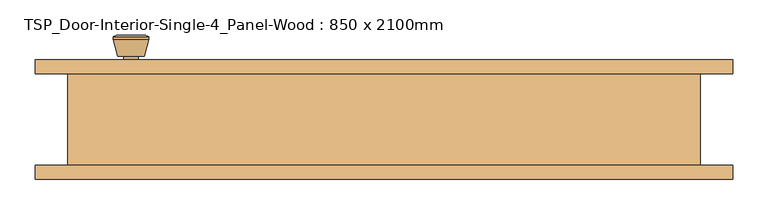
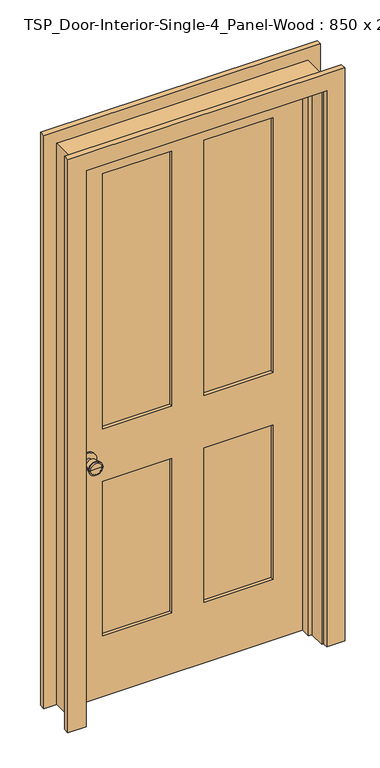
"""IFC4 building model written with IfcOpenShell, lengths in millimetres: door geometry, TSP_Door-Interior-Single-4_Panel-Wood : 850 x 2100mm."""

import ifcopenshell
import ifcopenshell.guid

model = None  # the IFC model being written
_history = None  # IfcOwnerHistory: only IFC2X3 demands one
_inside = {}  # id of a spatial element -> (the spatial element, [elements in it])
_under = {}  # id of a project, library or spatial element -> (it, [spatial elements below it])
_declared = {}  # id of a project -> (the project, [libraries it declares])
_typed = {}  # id of a type object -> (the type object, [elements of that type])
_made_of = {}  # id of a material, layer set ... -> (it, [elements and type objects made of it])


def new_model(schema):
    """Start an empty IFC model of exactly this schema.

    Asked for "IFC4X3", IfcOpenShell would pick the latest addendum, in which some entities
    have other attributes; the version numbers below select the first issue.
    IFC2X3 requires an IfcOwnerHistory on every rooted entity: one is made here for all.
    """
    global model, _history
    if schema == "IFC4X3":
        model = ifcopenshell.file(schema_version=(4, 3, 0, 0))
    else:
        model = ifcopenshell.file(schema=schema)
    _inside.clear()
    _under.clear()
    _declared.clear()
    _typed.clear()
    _made_of.clear()
    _history = None
    if model.schema == "IFC2X3":
        org = make("IfcOrganization", Name="unknown")
        user = make(
            "IfcPersonAndOrganization",
            ThePerson=make("IfcPerson", FamilyName="unknown"),
            TheOrganization=org,
        )
        app = make(
            "IfcApplication",
            ApplicationDeveloper=org,
            Version="unknown",
            ApplicationFullName="unknown",
            ApplicationIdentifier="unknown",
        )
        _history = make(
            "IfcOwnerHistory",
            OwningUser=user,
            OwningApplication=app,
            ChangeAction="ADDED",
            CreationDate=0,
        )
    return model


def make(cls, **values):
    """One entity of the class cls with the attributes given. An attribute that is None is left unset."""
    return model.create_entity(
        cls, **{name: value for name, value in values.items() if value is not None}
    )


def rooted(cls, **values):
    """An entity with a GlobalId (a new one), such as an element, a storey or a relation."""
    return make(cls, GlobalId=ifcopenshell.guid.new(), OwnerHistory=_history, **values)


def si_unit(unit_type, name, prefix=None):
    """IfcSIUnit, for example si_unit("LENGTHUNIT", "METRE", prefix="MILLI")."""
    return make("IfcSIUnit", UnitType=unit_type, Prefix=prefix, Name=name)


def assignment(units):
    """IfcUnitAssignment: the units of a project."""
    return None if units is None else make("IfcUnitAssignment", Units=units)


def point(xyz):
    """IfcCartesianPoint."""
    return None if xyz is None else make("IfcCartesianPoint", Coordinates=xyz)


def direction(xyz):
    """IfcDirection."""
    return None if xyz is None else make("IfcDirection", DirectionRatios=xyz)


def frame(location, z_axis=None, x_axis=None):
    """IfcAxis2Placement3D, a coordinate frame: its origin and axes. An axis left out is left unset."""
    return make(
        "IfcAxis2Placement3D",
        Location=point(location),
        Axis=direction(z_axis),
        RefDirection=direction(x_axis),
    )


def frame_2d(location, x_axis=None):
    """IfcAxis2Placement2D, a coordinate frame in the plane: its origin and x axis."""
    return make(
        "IfcAxis2Placement2D", Location=point(location), RefDirection=direction(x_axis)
    )


def origin():
    """The frame at (0, 0, 0) with its axes left unset."""
    return frame((0.0, 0.0, 0.0))


def place(relative_to, where):
    """IfcLocalPlacement: puts the frame where relative to a parent placement (None: the world)."""
    return make(
        "IfcLocalPlacement", PlacementRelTo=relative_to, RelativePlacement=where
    )


def context(
    kind, dimensions, precision=None, world=None, true_north=None, identifier=None
):
    """IfcGeometricRepresentationContext, for example the 3D "Model" context."""
    return make(
        "IfcGeometricRepresentationContext",
        ContextIdentifier=identifier,
        ContextType=kind,
        CoordinateSpaceDimension=dimensions,
        Precision=precision,
        WorldCoordinateSystem=world,
        TrueNorth=true_north,
    )


def project(units=None, contexts=None):
    """IfcProject with its units and contexts."""
    return rooted(
        "IfcProject",
        Name="project",
        RepresentationContexts=contexts,
        UnitsInContext=assignment(units),
    )


def spatial(cls, under=None, at=None, **own):
    """A site, building, storey or space (cls), placed at a placement, below another one or the project."""
    s = rooted(cls, ObjectPlacement=at, **own)
    if under is not None:
        _under.setdefault(under.id(), (under, []))[1].append(s)
    return s


def polyline(points):
    """IfcPolyline through the points."""
    return make("IfcPolyline", Points=[point(p) for p in points])


def circle_curve(where, radius):
    """IfcCircle in the frame where."""
    return make("IfcCircle", Position=where, Radius=radius)


def trimmed(basis, trim1, trim2, sense, master):
    """IfcTrimmedCurve: the piece of a basis curve between two trims."""
    return make(
        "IfcTrimmedCurve",
        BasisCurve=basis,
        Trim1=trim1,
        Trim2=trim2,
        SenseAgreement=sense,
        MasterRepresentation=master,
    )


def segment(curve, same_sense, transition):
    """IfcCompositeCurveSegment."""
    return make(
        "IfcCompositeCurveSegment",
        Transition=transition,
        SameSense=same_sense,
        ParentCurve=curve,
    )


def composite_curve(segments, self_intersect=None):
    """IfcCompositeCurve: segments joined end to end."""
    return make("IfcCompositeCurve", Segments=segments, SelfIntersect=self_intersect)


def outline(outer, holes=None, kind="AREA"):
    """IfcArbitraryClosedProfileDef: a profile drawn as a closed curve; with holes, ...WithVoids."""
    if holes is None:
        return make("IfcArbitraryClosedProfileDef", ProfileType=kind, OuterCurve=outer)
    return make(
        "IfcArbitraryProfileDefWithVoids",
        ProfileType=kind,
        OuterCurve=outer,
        InnerCurves=holes,
    )


def extrude(swept, where, along, depth):
    """IfcExtrudedAreaSolid: the profile swept, set in the frame where, extruded along a direction by depth."""
    return make(
        "IfcExtrudedAreaSolid",
        SweptArea=swept,
        Position=where,
        ExtrudedDirection=direction(along),
        Depth=depth,
    )


def faces_of(points, faces, orient=None, outer=None):
    """IfcFace entities. A face is a list of loops; a loop is a list of indices into points, from 0.

    orient and outer hold one flag for each loop. By default every Orientation is true, the
    first loop of a face is its IfcFaceOuterBound and the others are IfcFaceBound.
    """
    made = []
    for i, loops in enumerate(faces):
        bounds = []
        for j, loop in enumerate(loops):
            is_outer = j == 0 if outer is None else outer[i][j]
            bounds.append(
                make(
                    "IfcFaceOuterBound" if is_outer else "IfcFaceBound",
                    Bound=make("IfcPolyLoop", Polygon=[points[k] for k in loop]),
                    Orientation=True if orient is None else orient[i][j],
                )
            )
        made.append(make("IfcFace", Bounds=bounds))
    return made


def faceted_brep(points, faces, orient=None, outer=None, voids=None):
    """IfcFacetedBrep: a solid bounded by flat faces; with voids (closed shells), ...WithVoids."""
    shared = [point(p) for p in points]
    hull = make("IfcClosedShell", CfsFaces=faces_of(shared, faces, orient, outer))
    if voids is None:
        return make("IfcFacetedBrep", Outer=hull)
    return make(
        "IfcFacetedBrepWithVoids",
        Outer=hull,
        Voids=[
            make(cls, CfsFaces=faces_of(shared, fs, o, b)) for cls, fs, o, b in voids
        ],
    )


def shape(context_of_items, identifier, shape_type, items):
    """IfcShapeRepresentation: the items that make up one representation, for example the "Body"."""
    return make(
        "IfcShapeRepresentation",
        ContextOfItems=context_of_items,
        RepresentationIdentifier=identifier,
        RepresentationType=shape_type,
        Items=items,
    )


def source(mapping_origin, context_of_items, identifier, shape_type, items):
    """IfcRepresentationMap: a shape defined once, which mapped items show again and again."""
    return make(
        "IfcRepresentationMap",
        MappingOrigin=mapping_origin,
        MappedRepresentation=shape(context_of_items, identifier, shape_type, items),
    )


def transform(
    local_origin,
    x_axis=None,
    y_axis=None,
    z_axis=None,
    scale=None,
    scale2=None,
    scale3=None,
    uniform=True,
):
    """IfcCartesianTransformationOperator3D, or its non-uniform kind. x_axis, y_axis, z_axis: its Axis1, 2, 3."""
    if uniform:
        return make(
            "IfcCartesianTransformationOperator3D",
            Axis1=direction(x_axis),
            Axis2=direction(y_axis),
            LocalOrigin=point(local_origin),
            Scale=scale,
            Axis3=direction(z_axis),
        )
    return make(
        "IfcCartesianTransformationOperator3DnonUniform",
        Axis1=direction(x_axis),
        Axis2=direction(y_axis),
        LocalOrigin=point(local_origin),
        Scale=scale,
        Axis3=direction(z_axis),
        Scale2=scale2,
        Scale3=scale3,
    )


def mapped(mapping_source, mapping_target):
    """IfcMappedItem: shows the shape of a source again, moved by a transform."""
    return make(
        "IfcMappedItem", MappingSource=mapping_source, MappingTarget=mapping_target
    )


def made_of(thing, what):
    """Note that an element or type object is made of a material, layer set ...; save() writes the relation."""
    if what is not None:
        _made_of.setdefault(what.id(), (what, []))[1].append(thing)
    return thing


def element(
    cls,
    number,
    at=None,
    inside=None,
    cuts=None,
    type_object=None,
    material=None,
    context=None,
    identifier="Body",
    shape_type=None,
    held_by="IfcProductDefinitionShape",
    body=None,
    shapes=None,
    **own,
):
    """One element of the class cls, such as IfcWall. Its Tag is "e" and its number.

    at: its placement. inside: the storey or other place that contains it. cuts: it is an
    opening in that element (IfcRelVoidsElement). A single representation is given by context,
    identifier, shape_type and body (its items); several are given by shapes. held_by: the class
    of the entity that holds the representations. save() writes the other relations.
    """
    e = rooted(cls, Tag="e%d" % number, ObjectPlacement=at, **own)
    if body is not None:
        shapes = [shape(context, identifier, shape_type, body)]
    if shapes is not None:
        e.Representation = make(held_by, Representations=shapes)
    if inside is not None:
        _inside.setdefault(inside.id(), (inside, []))[1].append(e)
    if cuts is not None:
        rooted(
            "IfcRelVoidsElement", RelatingBuildingElement=cuts, RelatedOpeningElement=e
        )
    if type_object is not None:
        _typed.setdefault(type_object.id(), (type_object, []))[1].append(e)
    return made_of(e, material)


def aggregate(whole, parts):
    """IfcRelAggregates: a whole, such as a stair, and the parts it consists of."""
    return rooted("IfcRelAggregates", RelatingObject=whole, RelatedObjects=parts)


def save(model, path):
    """Write the relations noted so far, then the file.

    IfcRelAggregates (storeys below a building ...), IfcRelContainedInSpatialStructure (elements
    in a storey), IfcRelDefinesByType, IfcRelAssociatesMaterial and IfcRelDeclares: one each for
    every whole, place, type object, material and project.
    """
    for whole, parts in _under.values():
        aggregate(whole, parts)
    for where, things in _inside.values():
        rooted(
            "IfcRelContainedInSpatialStructure",
            RelatedElements=things,
            RelatingStructure=where,
        )
    for kind, things in _typed.values():
        rooted("IfcRelDefinesByType", RelatedObjects=things, RelatingType=kind)
    for what, things in _made_of.values():
        rooted("IfcRelAssociatesMaterial", RelatedObjects=things, RelatingMaterial=what)
    for by, libraries in _declared.values():
        rooted("IfcRelDeclares", RelatingContext=by, RelatedDefinitions=libraries)
    model.write(path)


def plane_surface(at):
    """IfcPlane: the flat surface through the origin of the frame at, square to its z axis."""
    return make("IfcPlane", Position=at)


def cylinder_surface(at, radius):
    """IfcCylindricalSurface: all points at the distance radius from the z axis of the frame at."""
    return make("IfcCylindricalSurface", Position=at, Radius=radius)


def revolved_surface(curve, axis_point, axis_direction):
    """IfcSurfaceOfRevolution: the curve turned about the line through axis_point along axis_direction."""
    return make(
        "IfcSurfaceOfRevolution",
        SweptCurve=make("IfcArbitraryOpenProfileDef", ProfileType="CURVE", Curve=curve),
        AxisPosition=make("IfcAxis1Placement", Location=point(axis_point), Axis=direction(axis_direction)),
    )


def advanced_brep(points, edges, surfaces, faces):
    """IfcAdvancedBrep: a solid bounded by faces that lie on surfaces and meet in shared edges.

    An edge is (start, end): straight between two places in points (the first is 0);
    or (start, end, curve); or (start, end, curve, False) where it runs against its curve.
    A face is (place in surfaces, loops), or (place, loops, False) where it looks against
    its surface's normal. A loop lists edges by number (the first is 1), with a minus sign
    where the edge is run from its end to its start. The first loop is the outer one.
    """
    corners = [point(p) for p in points]
    vertices = [make("IfcVertexPoint", VertexGeometry=c) for c in corners]
    made = []
    for start, end, *more in edges:
        made.append(
            make(
                "IfcEdgeCurve",
                EdgeStart=vertices[start],
                EdgeEnd=vertices[end],
                EdgeGeometry=more[0] if more else make("IfcPolyline", Points=[corners[start], corners[end]]),
                SameSense=more[1] if len(more) > 1 else True,
            )
        )
    hull = []
    for where, loops, *sense in faces:
        bounds = []
        for j, loop in enumerate(loops):
            ring = [make("IfcOrientedEdge", EdgeElement=made[abs(k) - 1], Orientation=k > 0) for k in loop]
            bounds.append(
                make(
                    "IfcFaceOuterBound" if j == 0 else "IfcFaceBound",
                    Bound=make("IfcEdgeLoop", EdgeList=ring),
                    Orientation=True,
                )
            )
        hull.append(make("IfcAdvancedFace", Bounds=bounds, FaceSurface=surfaces[where], SameSense=sense[0] if sense else True))
    return make("IfcAdvancedBrep", Outer=make("IfcClosedShell", CfsFaces=hull))


def tsp_door_interior_single_4_panel_wood_850_x_2100mm_ed8611a6(model_context):
    return source(origin(), model_context, "Body", "SolidModel", [
        advanced_brep(
        [(-360.0, 20.825, 914.4), (-350.0, 20.825, 914.4), (-370.0, 20.825, 914.4), (-339.5241324, -28.175, 914.4), (-360.0, -28.175, 914.4), (-380.4758676, -28.175, 914.4), (-335.0, -26.3471319, 914.4), (-385.0, -26.3471319, 914.4), (-335.0, -22.8834537, 914.4), (-385.0, -22.8834537, 914.4), (-341.363764, 1.825, 914.4), (-378.636236, 1.825, 914.4), (-350.0, 1.825, 914.4), (-370.0, 1.825, 914.4)],
        [
            (0, 1),
            (1, 2, circle_curve(frame((-360.0, 20.825, 914.4), z_axis=(0.0, 1.0, 0.0), x_axis=(-1.0, 0.0, 0.0)), 10.0)),
            (2, 0),
            (2, 1, circle_curve(frame((-360.0, 20.825, 914.4), z_axis=(0.0, 1.0, 0.0), x_axis=(-1.0, 0.0, 0.0)), 10.0)),
            (3, 4),
            (4, 5),
            (5, 3, circle_curve(frame((-360.0, -28.175, 914.4), z_axis=(0.0, -1.0, 0.0), x_axis=(-1.0, 0.0, 0.0)), 20.4758676)),
            (3, 5, circle_curve(frame((-360.0, -28.175, 914.4), z_axis=(0.0, -1.0, 0.0), x_axis=(-1.0, 0.0, 0.0)), 20.4758676)),
            (6, 3),
            (5, 7),
            (7, 6, circle_curve(frame((-360.0, -26.3471319, 914.4), z_axis=(0.0, -1.0, 0.0), x_axis=(-1.0, 0.0, 0.0)), 25.0)),
            (6, 7, circle_curve(frame((-360.0, -26.3471319, 914.4), z_axis=(0.0, -1.0, 0.0), x_axis=(-1.0, 0.0, 0.0)), 25.0)),
            (8, 6),
            (7, 9),
            (9, 8, circle_curve(frame((-360.0, -22.8834537, 914.4), z_axis=(0.0, -1.0, 0.0), x_axis=(-1.0, 0.0, 0.0)), 25.0)),
            (8, 9, circle_curve(frame((-360.0, -22.8834537, 914.4), z_axis=(0.0, -1.0, 0.0), x_axis=(-1.0, 0.0, 0.0)), 25.0)),
            (10, 8),
            (9, 11),
            (11, 10, circle_curve(frame((-360.0, 1.825, 914.4), z_axis=(0.0, -1.0, 0.0), x_axis=(-1.0, 0.0, 0.0)), 18.636236)),
            (10, 11, circle_curve(frame((-360.0, 1.825, 914.4), z_axis=(0.0, -1.0, 0.0), x_axis=(-1.0, 0.0, 0.0)), 18.636236)),
            (12, 10),
            (11, 13),
            (13, 12, circle_curve(frame((-360.0, 1.825, 914.4), z_axis=(0.0, -1.0, 0.0), x_axis=(-1.0, 0.0, 0.0)), 10.0)),
            (12, 13, circle_curve(frame((-360.0, 1.825, 914.4), z_axis=(0.0, -1.0, 0.0), x_axis=(-1.0, 0.0, 0.0)), 10.0)),
            (1, 12),
            (13, 2),
        ],
        [
            plane_surface(frame((-360.0, 20.825, 914.4), z_axis=(0.0, 1.0, 0.0), x_axis=(-1.0, 0.0, 0.0))),
            plane_surface(frame((-360.0, -28.175, 914.4), z_axis=(0.0, -1.0, 0.0), x_axis=(-1.0, 0.0, 0.0))),
            revolved_surface(polyline([(-380.4758676, -28.175, 914.4), (-385.0, -26.3471319, 914.4)]), (-360.0, 20.825, 914.4), (0.0, 1.0, 0.0)),
            cylinder_surface(frame((-360.0, 20.825, 914.4), z_axis=(0.0, 1.0, 0.0), x_axis=(-1.0, 0.0, 0.0)), 25.0),
            revolved_surface(polyline([(-385.0, -22.8834537, 914.4), (-378.636236, 1.825, 914.4)]), (-360.0, 20.825, 914.4), (0.0, 1.0, 0.0)),
            plane_surface(frame((-360.0, 1.825, 914.4), z_axis=(0.0, 1.0, 0.0), x_axis=(-1.0, 0.0, 0.0))),
            cylinder_surface(frame((-360.0, 20.825, 914.4), z_axis=(0.0, 1.0, 0.0), x_axis=(-1.0, 0.0, 0.0)), 10.0),
        ],
        [
            (0, [[1, 2, 3]]),
            (0, [[-3, 4, -1]]),
            (1, [[5, 6, 7]]),
            (1, [[-6, -5, 8]]),
            (2, [[9, -7, 10, 11]]),
            (2, [[-10, -8, -9, 12]]),
            (3, [[13, -11, 14, 15]]),
            (3, [[-14, -12, -13, 16]]),
            (4, [[17, -15, 18, 19]]),
            (4, [[-18, -16, -17, 20]]),
            (5, [[21, -19, 22, 23]]),
            (5, [[-22, -20, -21, 24]]),
            (6, [[25, -23, 26, -2]]),
            (6, [[-26, -24, -25, -4]]),
        ],
    ),
        extrude(outline(composite_curve([segment(trimmed(circle_curve(frame_2d((914.4, -360.0)), 30.0), [point((914.4, -390.0))], [point((914.4, -330.0))], False, "CARTESIAN"), True, "CONTINUOUS"), segment(trimmed(circle_curve(frame_2d((914.4, -360.0)), 30.0), [point((914.4, -330.0))], [point((914.4, -390.0))], False, "CARTESIAN"), True, "CONTINUOUS")], self_intersect=False)), frame((0.0, 20.825, 0.0), z_axis=(0.0, 1.0, 0.0), x_axis=(0.0, 0.0, 1.0)), (0.0, 0.0, 1.0), 6.0),
        advanced_brep(
        [(-360.0, 67.825, 914.4), (-370.0, 67.825, 914.4), (-350.0, 67.825, 914.4), (-339.5241324, 116.825, 914.4), (-380.4758676, 116.825, 914.4), (-360.0, 116.825, 914.4), (-335.0, 114.9971319, 914.4), (-385.0, 114.9971319, 914.4), (-335.0, 111.5334537, 914.4), (-385.0, 111.5334537, 914.4), (-341.363764, 86.825, 914.4), (-378.636236, 86.825, 914.4), (-350.0, 86.825, 914.4), (-370.0, 86.825, 914.4)],
        [
            (0, 1),
            (1, 2, circle_curve(frame((-360.0, 67.825, 914.4), z_axis=(0.0, -1.0, 0.0), x_axis=(-1.0, 0.0, 0.0)), 10.0)),
            (2, 0),
            (2, 1, circle_curve(frame((-360.0, 67.825, 914.4), z_axis=(0.0, -1.0, 0.0), x_axis=(-1.0, 0.0, 0.0)), 10.0)),
            (3, 4, circle_curve(frame((-360.0, 116.825, 914.4), z_axis=(0.0, 1.0, 0.0), x_axis=(-1.0, 0.0, 0.0)), 20.4758676)),
            (4, 5),
            (5, 3),
            (4, 3, circle_curve(frame((-360.0, 116.825, 914.4), z_axis=(0.0, 1.0, 0.0), x_axis=(-1.0, 0.0, 0.0)), 20.4758676)),
            (6, 7, circle_curve(frame((-360.0, 114.9971319, 914.4), z_axis=(0.0, 1.0, 0.0), x_axis=(-1.0, 0.0, 0.0)), 25.0)),
            (7, 4),
            (3, 6),
            (7, 6, circle_curve(frame((-360.0, 114.9971319, 914.4), z_axis=(0.0, 1.0, 0.0), x_axis=(-1.0, 0.0, 0.0)), 25.0)),
            (8, 9, circle_curve(frame((-360.0, 111.5334537, 914.4), z_axis=(0.0, 1.0, 0.0), x_axis=(-1.0, 0.0, 0.0)), 25.0)),
            (9, 7),
            (6, 8),
            (9, 8, circle_curve(frame((-360.0, 111.5334537, 914.4), z_axis=(0.0, 1.0, 0.0), x_axis=(-1.0, 0.0, 0.0)), 25.0)),
            (10, 11, circle_curve(frame((-360.0, 86.825, 914.4), z_axis=(0.0, 1.0, 0.0), x_axis=(-1.0, 0.0, 0.0)), 18.636236)),
            (11, 9),
            (8, 10),
            (11, 10, circle_curve(frame((-360.0, 86.825, 914.4), z_axis=(0.0, 1.0, 0.0), x_axis=(-1.0, 0.0, 0.0)), 18.636236)),
            (12, 13, circle_curve(frame((-360.0, 86.825, 914.4), z_axis=(0.0, 1.0, 0.0), x_axis=(-1.0, 0.0, 0.0)), 10.0)),
            (13, 11),
            (10, 12),
            (13, 12, circle_curve(frame((-360.0, 86.825, 914.4), z_axis=(0.0, 1.0, 0.0), x_axis=(-1.0, 0.0, 0.0)), 10.0)),
            (1, 13),
            (12, 2),
        ],
        [
            plane_surface(frame((-360.0, 67.825, 914.4), z_axis=(0.0, -1.0, 0.0), x_axis=(-1.0, 0.0, 0.0))),
            plane_surface(frame((-360.0, 116.825, 914.4), z_axis=(0.0, 1.0, 0.0), x_axis=(-1.0, 0.0, 0.0))),
            revolved_surface(polyline([(-380.4758676, 116.825, 914.4), (-385.0, 114.9971319, 914.4)]), (-360.0, 67.825, 914.4), (0.0, -1.0, 0.0)),
            cylinder_surface(frame((-360.0, 67.825, 914.4), z_axis=(0.0, -1.0, 0.0), x_axis=(-1.0, 0.0, 0.0)), 25.0),
            revolved_surface(polyline([(-385.0, 111.5334537, 914.4), (-378.636236, 86.825, 914.4)]), (-360.0, 67.825, 914.4), (0.0, -1.0, 0.0)),
            plane_surface(frame((-360.0, 86.825, 914.4), z_axis=(0.0, -1.0, 0.0), x_axis=(-1.0, 0.0, 0.0))),
            cylinder_surface(frame((-360.0, 67.825, 914.4), z_axis=(0.0, -1.0, 0.0), x_axis=(-1.0, 0.0, 0.0)), 10.0),
        ],
        [
            (0, [[1, 2, 3]]),
            (0, [[-3, 4, -1]]),
            (1, [[5, 6, 7]]),
            (1, [[8, -7, -6]]),
            (2, [[9, 10, -5, 11]]),
            (2, [[12, -11, -8, -10]]),
            (3, [[13, 14, -9, 15]]),
            (3, [[16, -15, -12, -14]]),
            (4, [[17, 18, -13, 19]]),
            (4, [[20, -19, -16, -18]]),
            (5, [[21, 22, -17, 23]]),
            (5, [[24, -23, -20, -22]]),
            (6, [[-2, 25, -21, 26]]),
            (6, [[-4, -26, -24, -25]]),
        ],
    ),
        extrude(outline(composite_curve([segment(trimmed(circle_curve(frame_2d((914.4, -360.0)), 30.0), [point((914.4, -390.0))], [point((914.4, -330.0))], False, "CARTESIAN"), True, "CONTINUOUS"), segment(trimmed(circle_curve(frame_2d((914.4, -360.0)), 30.0), [point((914.4, -330.0))], [point((914.4, -390.0))], False, "CARTESIAN"), True, "CONTINUOUS")], self_intersect=False)), frame((0.0, 61.825, 0.0), z_axis=(0.0, 1.0, 0.0), x_axis=(0.0, 0.0, 1.0)), (0.0, 0.0, 1.0), 6.0),
        faceted_brep([(450.0, 61.825, 0.0), (450.0, -68.175, 0.0), (425.0, -68.175, 0.0), (425.0, -8.1, 0.0), (412.3, -8.1, 0.0), (412.3, 26.825, 0.0), (425.0, 26.825, 0.0), (425.0, 61.825, 0.0), (450.0, 61.825, 2125.0), (450.0, -68.175, 2125.0), (-450.0, -68.175, 2125.0), (-450.0, -68.175, 0.0), (-425.0, -68.175, 0.0), (-425.0, -68.175, 2100.0), (425.0, -68.175, 2100.0), (425.0, -8.1, 2100.0), (-425.0, -8.1, 2100.0), (-425.0, -8.1, 0.0), (-412.3, -8.1, 0.0), (-412.3, -8.1, 2087.3), (412.3, -8.1, 2087.3), (412.3, 26.825, 2087.3), (-412.3, 26.825, 2087.3), (-412.3, 26.825, 0.0), (-425.0, 26.825, 0.0), (-425.0, 26.825, 2100.0), (425.0, 26.825, 2100.0), (425.0, 61.825, 2100.0), (-425.0, 61.825, 2100.0), (-425.0, 61.825, 0.0), (-450.0, 61.825, 0.0), (-450.0, 61.825, 2125.0)], [[[0, 1, 2, 3, 4, 5, 6, 7]], [[1, 0, 8, 9]], [[2, 1, 9, 10, 11, 12, 13, 14]], [[3, 2, 14, 15]], [[4, 3, 15, 16, 17, 18, 19, 20]], [[5, 4, 20, 21]], [[6, 5, 21, 22, 23, 24, 25, 26]], [[7, 6, 26, 27]], [[0, 7, 27, 28, 29, 30, 31, 8]], [[9, 8, 31, 10]], [[15, 14, 13, 16]], [[21, 20, 19, 22]], [[27, 26, 25, 28]], [[30, 29, 24, 23, 18, 17, 12, 11]], [[10, 31, 30, 11]], [[16, 13, 12, 17]], [[22, 19, 18, 23]], [[28, 25, 24, 29]]]),
        extrude(outline(polyline([(2100.0, -425.0), (0.0, -425.0), (0.0, 425.0), (2100.0, 425.0), (2100.0, -425.0)]), holes=[polyline([(1980.0, 57.5), (1980.0, 305.0), (1014.4, 305.0), (1014.4, 57.5), (1980.0, 57.5)]), polyline([(1014.4, -57.5), (1014.4, -305.0), (1980.0, -305.0), (1980.0, -57.5), (1014.4, -57.5)]), polyline([(814.4, 57.5), (814.4, 305.0), (230.0, 305.0), (230.0, 57.5), (814.4, 57.5)]), polyline([(230.0, -57.5), (230.0, -305.0), (814.4, -305.0), (814.4, -57.5), (230.0, -57.5)])]), frame((0.0, 26.825, 0.0), z_axis=(0.0, 1.0, 0.0), x_axis=(0.0, 0.0, 1.0)), (0.0, 0.0, 1.0), 35.0),
        extrude(outline(polyline([(305.0, 38.4916667), (57.5, 38.4916667), (57.5, 50.1583333), (305.0, 50.1583333), (305.0, 38.4916667)])), frame((0.0, 0.0, 1014.4), z_axis=(0.0, 0.0, 1.0), x_axis=(1.0, 0.0, 0.0)), (0.0, 0.0, 1.0), 965.6),
        extrude(outline(polyline([(-57.5, 38.4916667), (-305.0, 38.4916667), (-305.0, 50.1583333), (-57.5, 50.1583333), (-57.5, 38.4916667)])), frame((0.0, 0.0, 1014.4), z_axis=(0.0, 0.0, 1.0), x_axis=(1.0, 0.0, 0.0)), (0.0, 0.0, 1.0), 965.6),
        extrude(outline(polyline([(305.0, 38.4916667), (57.5, 38.4916667), (57.5, 50.1583333), (305.0, 50.1583333), (305.0, 38.4916667)])), frame((0.0, 0.0, 230.0), z_axis=(0.0, 0.0, 1.0), x_axis=(1.0, 0.0, 0.0)), (0.0, 0.0, 1.0), 584.4),
        extrude(outline(polyline([(-57.5, 38.4916667), (-305.0, 38.4916667), (-305.0, 50.1583333), (-57.5, 50.1583333), (-57.5, 38.4916667)])), frame((0.0, 0.0, 230.0), z_axis=(0.0, 0.0, 1.0), x_axis=(1.0, 0.0, 0.0)), (0.0, 0.0, 1.0), 584.4),
        extrude(outline(polyline([(0.0, 431.35), (0.0, 496.35), (2171.35, 496.35), (2171.35, -496.35), (0.0, -496.35), (0.0, -431.35), (2106.35, -431.35), (2106.35, 431.35), (0.0, 431.35)])), frame((0.0, 61.825, 0.0), z_axis=(0.0, 1.0, 0.0), x_axis=(0.0, 0.0, 1.0)), (0.0, 0.0, 1.0), 20.0),
        extrude(outline(polyline([(0.0, 431.35), (0.0, 496.35), (2171.35, 496.35), (2171.35, -496.35), (0.0, -496.35), (0.0, -431.35), (2106.35, -431.35), (2106.35, 431.35), (0.0, 431.35)])), frame((0.0, -88.175, 0.0), z_axis=(0.0, 1.0, 0.0), x_axis=(0.0, 0.0, 1.0)), (0.0, 0.0, 1.0), 20.0),
    ])


if __name__ == "__main__":
    model = new_model("IFC4")
    model_context = context("Model", 3, world=origin())
    ifc_project = project(units=[si_unit("LENGTHUNIT", "METRE", prefix="MILLI")], contexts=[model_context])
    site = spatial("IfcSite", under=ifc_project)
    building = spatial("IfcBuilding", under=site)
    placement = place(None, origin())
    tsp_door_interior_single_4_panel_wood_850_x_2100mm_shape = tsp_door_interior_single_4_panel_wood_850_x_2100mm_ed8611a6(model_context)
    element("IfcDoor", 1, ObjectType="TSP_Door-Interior-Single-4_Panel-Wood : 850 x 2100mm", at=placement, inside=building, context=model_context, shape_type="MappedRepresentation", body=[
        mapped(tsp_door_interior_single_4_panel_wood_850_x_2100mm_shape, transform((0.0, 0.0, 0.0), x_axis=(1.0, 0.0, 0.0), y_axis=(0.0, 1.0, 0.0), z_axis=(0.0, 0.0, 1.0))),
    ])
    save(model, "model.ifc")

# Revit data of these elements
# Type "TSP_Door-Interior-Single-4_Panel-Wood : 850 x 2100mm"
#   Model = "TSP_DOOR02W"
#   Type Mark = "243"
#   Assembly Code = "C1020300"
#   Analytic Construction = "Wooden"
#   Top Rail = 120 mm
#   Thickness = 35 mm
#   Thermal Resistance (R) = 0.455703 (m²·K)/W
#   Swing Angle [instance default] = 90.00°
#   Stiles = 120 mm
#   Rough Width = 900 mm
#   Rough Height = 2125 mm
#   Mullion = 115 mm
#   Lock Rail = 200 mm
#   Height = 2100 mm
#   Width = 850 mm
#   Heat Transfer Coefficient (U) = 2.19465 W/(m²·K)
#   Bottom Rail = 230 mm
#   Define Thermal Properties by = 1
#   Trim Material = Cherry
#   Panel Material = Cherry
#   Frame Material = Cherry
#   Door Handle Material = Aluminum
#   Visual Light Transmittance = 0
#   Solar Heat Gain Coefficient = 0
#   Wall Closure = (empty or 0)
#   Function = (empty or 0)
# Element 1 (IfcDoor, "TSP_Door-Interior-Single-4_Panel-Wood : 850 x 2100mm")
#   Materials on its faces: "Cherry", "Aluminum"
# Materials
#   "Cherry": class "Wood", colour RGB 226 177 128, transparency 0, Description = "Prunus Serotina", Cost = 0
#   "Aluminum": class "Metal", colour RGB 247 247 247, transparency 0, Description = "Aluminum 6061", Cost = 0
